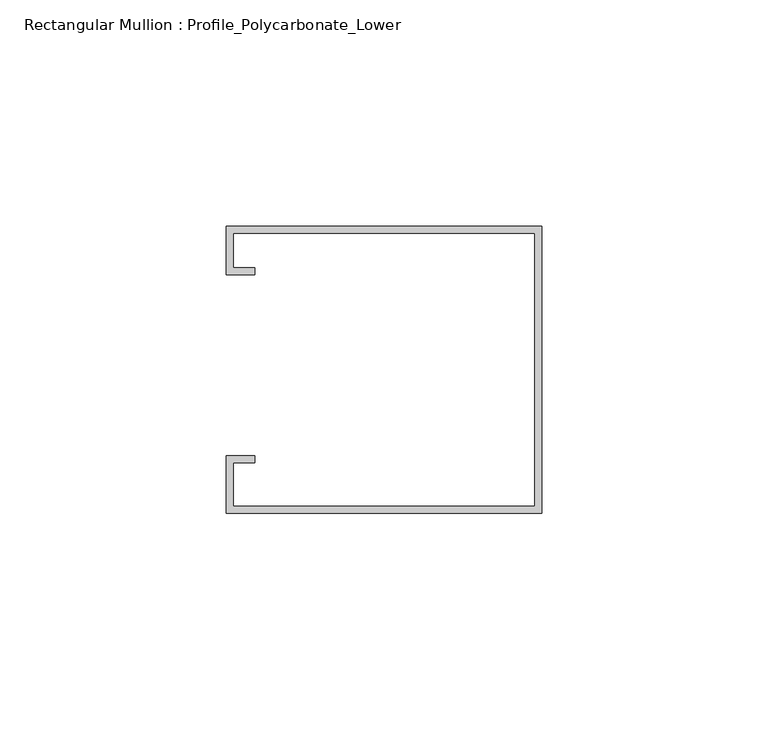
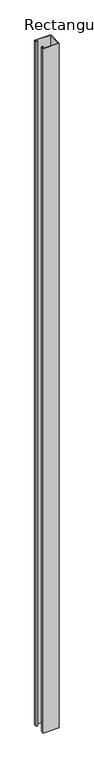
"""IFC4 building model written with IfcOpenShell, lengths in millimetres: member geometry, Rectangular Mullion : Profile_Polycarbonate_Lower."""

import ifcopenshell
import ifcopenshell.guid

model = None  # the IFC model being written
_history = None  # IfcOwnerHistory: only IFC2X3 demands one
_inside = {}  # id of a spatial element -> (the spatial element, [elements in it])
_under = {}  # id of a project, library or spatial element -> (it, [spatial elements below it])
_declared = {}  # id of a project -> (the project, [libraries it declares])
_typed = {}  # id of a type object -> (the type object, [elements of that type])
_made_of = {}  # id of a material, layer set ... -> (it, [elements and type objects made of it])


def new_model(schema):
    """Start an empty IFC model of exactly this schema.

    Asked for "IFC4X3", IfcOpenShell would pick the latest addendum, in which some entities
    have other attributes; the version numbers below select the first issue.
    IFC2X3 requires an IfcOwnerHistory on every rooted entity: one is made here for all.
    """
    global model, _history
    if schema == "IFC4X3":
        model = ifcopenshell.file(schema_version=(4, 3, 0, 0))
    else:
        model = ifcopenshell.file(schema=schema)
    _inside.clear()
    _under.clear()
    _declared.clear()
    _typed.clear()
    _made_of.clear()
    _history = None
    if model.schema == "IFC2X3":
        org = make("IfcOrganization", Name="unknown")
        user = make(
            "IfcPersonAndOrganization",
            ThePerson=make("IfcPerson", FamilyName="unknown"),
            TheOrganization=org,
        )
        app = make(
            "IfcApplication",
            ApplicationDeveloper=org,
            Version="unknown",
            ApplicationFullName="unknown",
            ApplicationIdentifier="unknown",
        )
        _history = make(
            "IfcOwnerHistory",
            OwningUser=user,
            OwningApplication=app,
            ChangeAction="ADDED",
            CreationDate=0,
        )
    return model


def make(cls, **values):
    """One entity of the class cls with the attributes given. An attribute that is None is left unset."""
    return model.create_entity(
        cls, **{name: value for name, value in values.items() if value is not None}
    )


def rooted(cls, **values):
    """An entity with a GlobalId (a new one), such as an element, a storey or a relation."""
    return make(cls, GlobalId=ifcopenshell.guid.new(), OwnerHistory=_history, **values)


def si_unit(unit_type, name, prefix=None):
    """IfcSIUnit, for example si_unit("LENGTHUNIT", "METRE", prefix="MILLI")."""
    return make("IfcSIUnit", UnitType=unit_type, Prefix=prefix, Name=name)


def assignment(units):
    """IfcUnitAssignment: the units of a project."""
    return None if units is None else make("IfcUnitAssignment", Units=units)


def point(xyz):
    """IfcCartesianPoint."""
    return None if xyz is None else make("IfcCartesianPoint", Coordinates=xyz)


def direction(xyz):
    """IfcDirection."""
    return None if xyz is None else make("IfcDirection", DirectionRatios=xyz)


def frame(location, z_axis=None, x_axis=None):
    """IfcAxis2Placement3D, a coordinate frame: its origin and axes. An axis left out is left unset."""
    return make(
        "IfcAxis2Placement3D",
        Location=point(location),
        Axis=direction(z_axis),
        RefDirection=direction(x_axis),
    )


def origin():
    """The frame at (0, 0, 0) with its axes left unset."""
    return frame((0.0, 0.0, 0.0))


def place(relative_to, where):
    """IfcLocalPlacement: puts the frame where relative to a parent placement (None: the world)."""
    return make(
        "IfcLocalPlacement", PlacementRelTo=relative_to, RelativePlacement=where
    )


def context(
    kind, dimensions, precision=None, world=None, true_north=None, identifier=None
):
    """IfcGeometricRepresentationContext, for example the 3D "Model" context."""
    return make(
        "IfcGeometricRepresentationContext",
        ContextIdentifier=identifier,
        ContextType=kind,
        CoordinateSpaceDimension=dimensions,
        Precision=precision,
        WorldCoordinateSystem=world,
        TrueNorth=true_north,
    )


def project(units=None, contexts=None):
    """IfcProject with its units and contexts."""
    return rooted(
        "IfcProject",
        Name="project",
        RepresentationContexts=contexts,
        UnitsInContext=assignment(units),
    )


def spatial(cls, under=None, at=None, **own):
    """A site, building, storey or space (cls), placed at a placement, below another one or the project."""
    s = rooted(cls, ObjectPlacement=at, **own)
    if under is not None:
        _under.setdefault(under.id(), (under, []))[1].append(s)
    return s


def polyline(points):
    """IfcPolyline through the points."""
    return make("IfcPolyline", Points=[point(p) for p in points])


def outline(outer, holes=None, kind="AREA"):
    """IfcArbitraryClosedProfileDef: a profile drawn as a closed curve; with holes, ...WithVoids."""
    if holes is None:
        return make("IfcArbitraryClosedProfileDef", ProfileType=kind, OuterCurve=outer)
    return make(
        "IfcArbitraryProfileDefWithVoids",
        ProfileType=kind,
        OuterCurve=outer,
        InnerCurves=holes,
    )


def extrude(swept, where, along, depth):
    """IfcExtrudedAreaSolid: the profile swept, set in the frame where, extruded along a direction by depth."""
    return make(
        "IfcExtrudedAreaSolid",
        SweptArea=swept,
        Position=where,
        ExtrudedDirection=direction(along),
        Depth=depth,
    )


def shape(context_of_items, identifier, shape_type, items):
    """IfcShapeRepresentation: the items that make up one representation, for example the "Body"."""
    return make(
        "IfcShapeRepresentation",
        ContextOfItems=context_of_items,
        RepresentationIdentifier=identifier,
        RepresentationType=shape_type,
        Items=items,
    )


def source(mapping_origin, context_of_items, identifier, shape_type, items):
    """IfcRepresentationMap: a shape defined once, which mapped items show again and again."""
    return make(
        "IfcRepresentationMap",
        MappingOrigin=mapping_origin,
        MappedRepresentation=shape(context_of_items, identifier, shape_type, items),
    )


def transform(
    local_origin,
    x_axis=None,
    y_axis=None,
    z_axis=None,
    scale=None,
    scale2=None,
    scale3=None,
    uniform=True,
):
    """IfcCartesianTransformationOperator3D, or its non-uniform kind. x_axis, y_axis, z_axis: its Axis1, 2, 3."""
    if uniform:
        return make(
            "IfcCartesianTransformationOperator3D",
            Axis1=direction(x_axis),
            Axis2=direction(y_axis),
            LocalOrigin=point(local_origin),
            Scale=scale,
            Axis3=direction(z_axis),
        )
    return make(
        "IfcCartesianTransformationOperator3DnonUniform",
        Axis1=direction(x_axis),
        Axis2=direction(y_axis),
        LocalOrigin=point(local_origin),
        Scale=scale,
        Axis3=direction(z_axis),
        Scale2=scale2,
        Scale3=scale3,
    )


def mapped(mapping_source, mapping_target):
    """IfcMappedItem: shows the shape of a source again, moved by a transform."""
    return make(
        "IfcMappedItem", MappingSource=mapping_source, MappingTarget=mapping_target
    )


def made_of(thing, what):
    """Note that an element or type object is made of a material, layer set ...; save() writes the relation."""
    if what is not None:
        _made_of.setdefault(what.id(), (what, []))[1].append(thing)
    return thing


def element(
    cls,
    number,
    at=None,
    inside=None,
    cuts=None,
    type_object=None,
    material=None,
    context=None,
    identifier="Body",
    shape_type=None,
    held_by="IfcProductDefinitionShape",
    body=None,
    shapes=None,
    **own,
):
    """One element of the class cls, such as IfcWall. Its Tag is "e" and its number.

    at: its placement. inside: the storey or other place that contains it. cuts: it is an
    opening in that element (IfcRelVoidsElement). A single representation is given by context,
    identifier, shape_type and body (its items); several are given by shapes. held_by: the class
    of the entity that holds the representations. save() writes the other relations.
    """
    e = rooted(cls, Tag="e%d" % number, ObjectPlacement=at, **own)
    if body is not None:
        shapes = [shape(context, identifier, shape_type, body)]
    if shapes is not None:
        e.Representation = make(held_by, Representations=shapes)
    if inside is not None:
        _inside.setdefault(inside.id(), (inside, []))[1].append(e)
    if cuts is not None:
        rooted(
            "IfcRelVoidsElement", RelatingBuildingElement=cuts, RelatedOpeningElement=e
        )
    if type_object is not None:
        _typed.setdefault(type_object.id(), (type_object, []))[1].append(e)
    return made_of(e, material)


def aggregate(whole, parts):
    """IfcRelAggregates: a whole, such as a stair, and the parts it consists of."""
    return rooted("IfcRelAggregates", RelatingObject=whole, RelatedObjects=parts)


def save(model, path):
    """Write the relations noted so far, then the file.

    IfcRelAggregates (storeys below a building ...), IfcRelContainedInSpatialStructure (elements
    in a storey), IfcRelDefinesByType, IfcRelAssociatesMaterial and IfcRelDeclares: one each for
    every whole, place, type object, material and project.
    """
    for whole, parts in _under.values():
        aggregate(whole, parts)
    for where, things in _inside.values():
        rooted(
            "IfcRelContainedInSpatialStructure",
            RelatedElements=things,
            RelatingStructure=where,
        )
    for kind, things in _typed.values():
        rooted("IfcRelDefinesByType", RelatedObjects=things, RelatingType=kind)
    for what, things in _made_of.values():
        rooted("IfcRelAssociatesMaterial", RelatedObjects=things, RelatingMaterial=what)
    for by, libraries in _declared.values():
        rooted("IfcRelDeclares", RelatingContext=by, RelatedDefinitions=libraries)
    model.write(path)


def rectangular_mullion_profile_polycarbonate_lower_e256f0d7(model_context):
    return source(origin(), model_context, "Body", "SweptSolid", [
        extrude(outline(polyline([(0.0, -32.7), (-69.85, -32.7), (-69.85, -20.0), (-63.5, -20.0), (-63.5, -21.5875), (-68.2625, -21.5875), (-68.2625, -31.1125), (-1.5875, -31.1125), (-1.5875, 29.2125), (-68.2625, 29.2125), (-68.2625, 21.5875), (-63.5, 21.5875), (-63.5, 20.0), (-69.85, 20.0), (-69.85, 30.8), (0.0, 30.8), (0.0, -32.7)])), frame((0.0, 0.0, -3136.9), z_axis=(0.0, 0.0, 1.0), x_axis=(1.0, 0.0, 0.0)), (0.0, 0.0, 1.0), 3136.9),
    ])


if __name__ == "__main__":
    model = new_model("IFC4")
    model_context = context("Model", 3, world=origin())
    ifc_project = project(units=[si_unit("LENGTHUNIT", "METRE", prefix="MILLI")], contexts=[model_context])
    site = spatial("IfcSite", under=ifc_project)
    building = spatial("IfcBuilding", under=site)
    placement = place(None, origin())
    rectangular_mullion_profile_polycarbonate_lower_shape = rectangular_mullion_profile_polycarbonate_lower_e256f0d7(model_context)
    element("IfcMember", 1, ObjectType="Rectangular Mullion : Profile_Polycarbonate_Lower", at=placement, inside=building, context=model_context, shape_type="MappedRepresentation", body=[
        mapped(rectangular_mullion_profile_polycarbonate_lower_shape, transform((0.0, 0.0, 0.0), x_axis=(1.0, 0.0, 0.0), y_axis=(0.0, 1.0, 0.0), z_axis=(0.0, 0.0, 1.0))),
    ])
    save(model, "model.ifc")

# Revit data of these elements
# Type "Rectangular Mullion : Profile_Polycarbonate_Lower"
#   built-in parameter 1007322 = 0.208333 (stored number, unit not read)
#   built-in parameter 1007321 = 0 (stored number, unit not read)
#   built-in parameter 1007320 = 0.00520833 (stored number, unit not read)
# Element 1 (IfcMember, "Rectangular Mullion : Profile_Polycarbonate_Lower")
#   Materials on its faces: "ALUMINUM PROFILE AT POLYCARBONATE PANEL"
# Materials
#   "ALUMINUM PROFILE AT POLYCARBONATE PANEL": class "Metal", colour RGB 244 244 244, transparency 0, Description = "Aluminum 6061", Cost = 0
